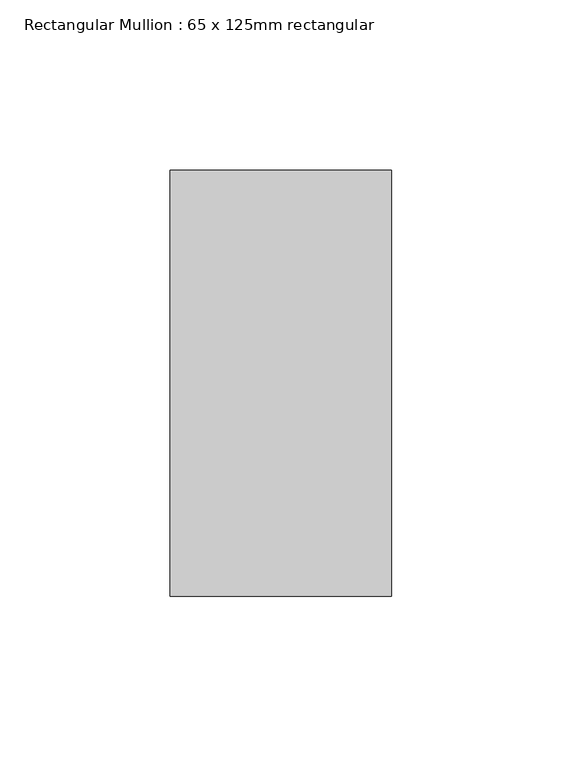
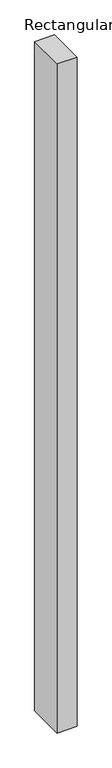
"""IFC4 building model written with IfcOpenShell, lengths in millimetres: member geometry, Rectangular Mullion : 65 x 125mm rectangular."""

from ifc_helpers import new_model, si_unit, frame, origin, place, context, project, spatial, polyline, outline, extrude, source, transform, mapped, element, save


def rectangular_mullion_65_x_125mm_rectangular_4f7d984b(model_context):
    return source(origin(), model_context, "Body", "SweptSolid", [
        extrude(outline(polyline([(0.0, 62.5), (0.0, -62.5), (-65.0, -62.5), (-65.0, 62.5), (0.0, 62.5)])), frame((0.0, 0.0, -2291.9433297), z_axis=(0.0, 0.0, 1.0), x_axis=(1.0, 0.0, 0.0)), (0.0, 0.0, 1.0), 2291.9433297),
    ])


if __name__ == "__main__":
    model = new_model("IFC4")
    model_context = context("Model", 3, world=origin())
    ifc_project = project(units=[si_unit("LENGTHUNIT", "METRE", prefix="MILLI")], contexts=[model_context])
    site = spatial("IfcSite", under=ifc_project)
    building = spatial("IfcBuilding", under=site)
    placement = place(None, origin())
    rectangular_mullion_65_x_125mm_rectangular_shape = rectangular_mullion_65_x_125mm_rectangular_4f7d984b(model_context)
    element("IfcMember", 1, ObjectType="Rectangular Mullion : 65 x 125mm rectangular", at=placement, inside=building, context=model_context, shape_type="MappedRepresentation", body=[
        mapped(rectangular_mullion_65_x_125mm_rectangular_shape, transform((0.0, 0.0, 0.0), x_axis=(1.0, 0.0, 0.0), y_axis=(0.0, 1.0, 0.0), z_axis=(0.0, 0.0, 1.0))),
    ])
    save(model, "model.ifc")

# Revit data of these elements
# Type "Rectangular Mullion : 65 x 125mm rectangular"
#   built-in parameter 1007304 = 0.410105 (stored number, unit not read)
#   built-in parameter 1007301 = 0.106627 (stored number, unit not read)
#   built-in parameter 1007300 = 0.106627 (stored number, unit not read)
# Element 1 (IfcMember, "Rectangular Mullion : 65 x 125mm rectangular")
#   Materials on its faces: "Aluminum"
# Materials
#   "Aluminum": class "Metal", colour RGB 244 245 246, transparency 0, Description = "Aluminum 6061", Cost = 0
